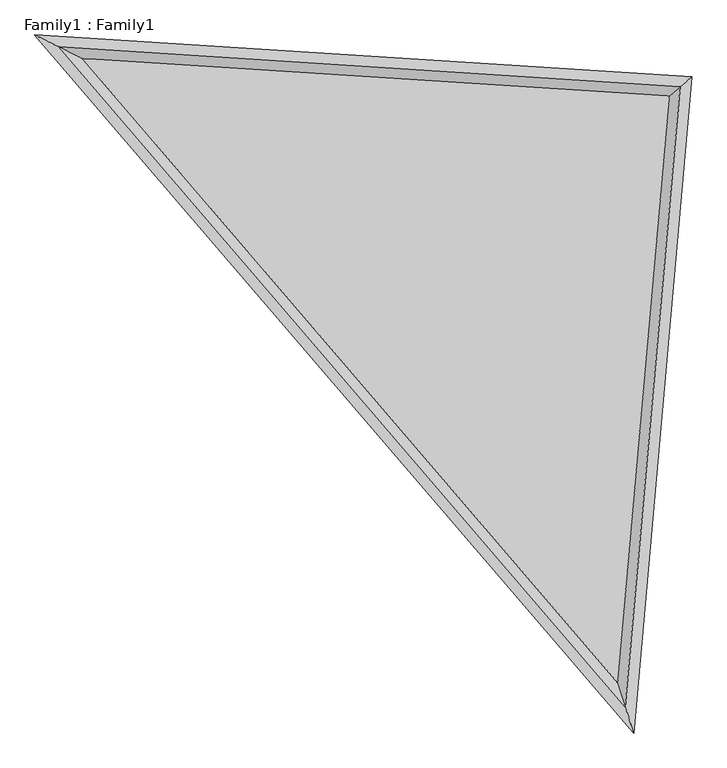
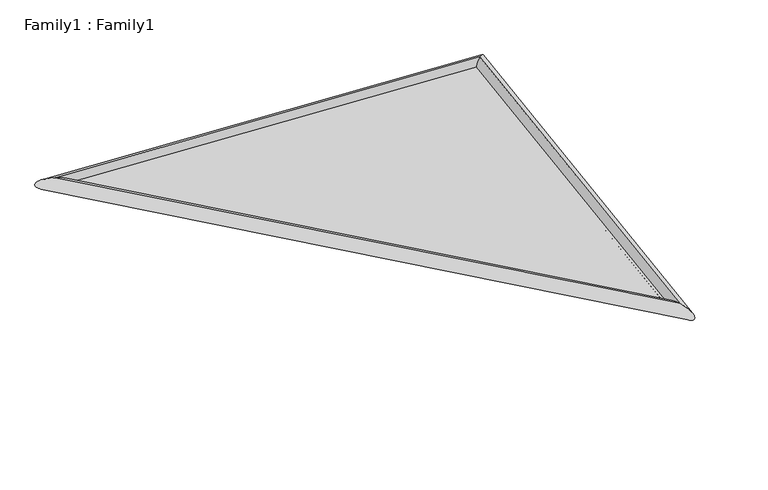
"""IFC4 building model written with IfcOpenShell, lengths in millimetres: proxy geometry, Family1 : Family1."""

from ifc_helpers import new_model, si_unit, frame, origin, origin_with_axes, place, context, project, spatial, polyline, ellipse_curve, outline, extrude, source, transform, mapped, element, save
from ifc_brep_helpers import cylinder_surface, advanced_brep


def family1_family1_131992ef(model_context):
    return source(origin(), model_context, "Body", "SolidModel", [
        extrude(outline(polyline([(2550.0361314, -3612.7426703), (-2857.7474921, 2688.1097571), (3074.6338117, 2308.5741181), (2550.0361314, -3612.7426703)])), origin_with_axes(), (0.0, 0.0, 1.0), 34.1328789),
        advanced_brep(
        [(2550.0361314, -3612.7426703, 100.0), (2550.0361314, -3612.7426703, -100.0), (-2857.7474921, 2688.1097571, -100.0), (-2857.7474921, 2688.1097571, 100.0), (3074.6338117, 2308.5741181, -100.0), (3074.6338117, 2308.5741181, 100.0)],
        [
            (0, 1, ellipse_curve(frame((2550.0361314, -3612.7426703, 0.0), z_axis=(-0.9521951064847551, -0.3054905549873608, 0.0), x_axis=(0.30549055498736083, -0.9521951064847552, 0.0)), 257.5135809, 100.0)),
            (1, 2),
            (2, 3, ellipse_curve(frame((-2857.7474921, 2688.1097571, 0.0), z_axis=(-0.446372539721607, -0.8948472248280609, 0.0), x_axis=(0.8948472248280611, -0.4463725397216071, 0.0)), 257.5135809, 100.0)),
            (3, 0),
            (1, 0, ellipse_curve(frame((2550.0361314, -3612.7426703, 0.0), z_axis=(-0.9521951064847551, -0.3054905549873608, 0.0), x_axis=(0.30549055498736083, -0.9521951064847552, 0.0)), 257.5135809, 100.0)),
            (3, 2, ellipse_curve(frame((-2857.7474921, 2688.1097571, 0.0), z_axis=(-0.446372539721607, -0.8948472248280609, 0.0), x_axis=(0.8948472248280611, -0.4463725397216071, 0.0)), 257.5135809, 100.0)),
            (2, 4),
            (4, 5, ellipse_curve(frame((3074.6338117, 2308.5741181, 0.0), z_axis=(-0.6512809022800948, 0.7588367323246981, 0.0), x_axis=(-0.7588367323246982, -0.6512809022800948, 0.0)), 143.1841912, 100.0)),
            (5, 3),
            (5, 4, ellipse_curve(frame((3074.6338117, 2308.5741181, 0.0), z_axis=(-0.6512809022800948, 0.7588367323246981, 0.0), x_axis=(-0.7588367323246982, -0.6512809022800948, 0.0)), 143.1841912, 100.0)),
            (4, 1),
            (0, 5),
        ],
        [
            cylinder_surface(frame((2550.0361314, -3612.7426703, 0.0), z_axis=(0.6512809022800864, -0.7588367323247055, 0.0), x_axis=(-0.7588367323247055, -0.6512809022800864, 0.0)), 100.0),
            cylinder_surface(frame((-2857.7474921, 2688.1097571, 0.0), z_axis=(-0.9979597362273316, 0.0638464162586658, 0.0), x_axis=(0.0638464162586658, 0.9979597362273316, 0.0)), 100.0),
            cylinder_surface(frame((3074.6338117, 2308.5741181, 0.0), z_axis=(0.0882491087109102, 0.9960984363062367, 0.0), x_axis=(0.9960984363062367, -0.0882491087109102, 0.0)), 100.0),
        ],
        [
            (0, [[1, 2, 3, 4]]),
            (0, [[5, -4, 6, -2]]),
            (1, [[-3, 7, 8, 9]]),
            (1, [[-6, -9, 10, -7]]),
            (2, [[-8, 11, -1, 12]]),
            (2, [[-10, -12, -5, -11]]),
        ],
    ),
    ])


if __name__ == "__main__":
    model = new_model("IFC4")
    model_context = context("Model", 3, world=origin())
    ifc_project = project(units=[si_unit("LENGTHUNIT", "METRE", prefix="MILLI")], contexts=[model_context])
    site = spatial("IfcSite", under=ifc_project)
    building = spatial("IfcBuilding", under=site)
    placement = place(None, origin())
    family1_family1_shape = family1_family1_131992ef(model_context)
    element("IfcBuildingElementProxy", 1, Name="Family1 : Family1", ObjectType="Family1 : Family1", at=placement, inside=building, context=model_context, shape_type="MappedRepresentation", body=[
        mapped(family1_family1_shape, transform((0.0, 0.0, 0.0), x_axis=(1.0, 0.0, 0.0), y_axis=(0.0, 1.0, 0.0), z_axis=(0.0, 0.0, 1.0))),
    ])
    save(model, "model.ifc")

# Revit data of these elements
# Type "Family1 : Family1"
#   Default Elevation = 0
# Element 1 (IfcBuildingElementProxy, "Family1 : Family1")
#   Materials on its faces: "Glass"
# Materials
#   "Glass": class "Glass", colour RGB 0 128 192, transparency 0.9, Description = "Soda Lime Glass", Cost = 0
